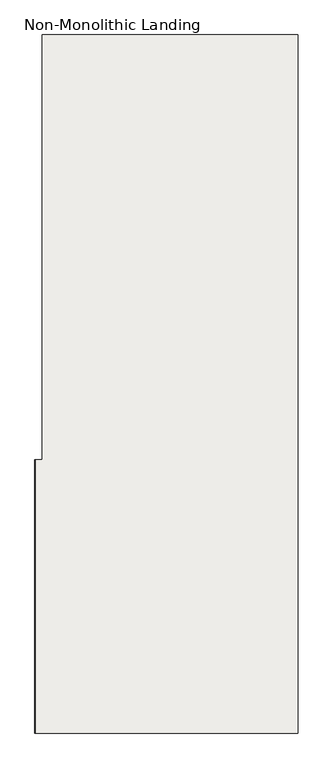
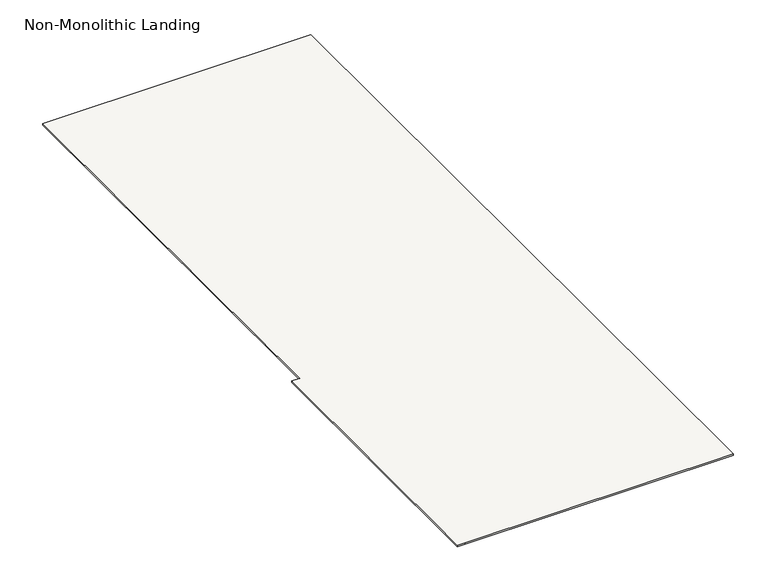
"""IFC4 building model written with IfcOpenShell, lengths in millimetres: slab geometry, Non-Monolithic Landing."""

from ifc_helpers import new_model, si_unit, origin, place, context, project, spatial, faceted_brep, source, transform, mapped, element, save


def non_monolithic_landing_37a11202(model_context):
    return source(origin(), model_context, "Body", "Brep", [
        faceted_brep([(-13356.0599092, 11395.4345331, 28470.5882353), (-13356.9099092, 11395.4345331, 28464.5882353), (-13356.9099092, 10220.4345331, 28464.5882353), (-13356.0599092, 10220.4345331, 28470.5882353), (-13325.0, 12030.4345331, 28470.5882353), (-13325.0, 11395.4345331, 28470.5882353), (-13325.0, 10220.4345331, 28470.5882353), (-12225.0, 10220.4345331, 28470.5882353), (-12225.0, 13220.4345331, 28470.5882353), (-13325.0, 13220.4345331, 28470.5882353), (-13325.0, 11395.4345331, 28464.5882353), (-13325.0, 12030.4345331, 28464.5882353), (-13324.15, 12030.4345331, 28464.5882353), (-13324.15, 13220.4345331, 28464.5882353), (-12225.0, 13220.4345331, 28464.5882353), (-12225.0, 10220.4345331, 28464.5882353), (-13325.0, 10220.4345331, 28464.5882353)], [[[0, 1, 2, 3]], [[4, 5, 0, 3, 6, 7, 8, 9]], [[10, 11, 12, 13, 14, 15, 16, 2, 1]], [[5, 4, 11, 10]], [[0, 5, 10, 1]], [[6, 3, 2, 16]], [[7, 6, 16, 15]], [[8, 7, 15, 14]], [[9, 8, 14, 13]], [[4, 12, 11]], [[12, 4, 9, 13]]]),
    ])


if __name__ == "__main__":
    model = new_model("IFC4")
    model_context = context("Model", 3, world=origin())
    ifc_project = project(units=[si_unit("LENGTHUNIT", "METRE", prefix="MILLI")], contexts=[model_context])
    site = spatial("IfcSite", under=ifc_project)
    building = spatial("IfcBuilding", under=site)
    placement = place(None, origin())
    non_monolithic_landing_shape = non_monolithic_landing_37a11202(model_context)
    element("IfcSlab", 1, ObjectType="Non-Monolithic Landing", at=placement, inside=building, context=model_context, shape_type="MappedRepresentation", body=[
        mapped(non_monolithic_landing_shape, transform((0.0, 0.0, 0.0), x_axis=(1.0, 0.0, 0.0), y_axis=(0.0, 1.0, 0.0), z_axis=(0.0, 0.0, 1.0))),
    ])
    save(model, "model.ifc")

# Revit data of these elements
# Element 1 (IfcSlab, "Non-Monolithic Landing")
#   Materials on its faces: "Steel, Paint Finish, Dark Gray"
# Materials
#   "Steel, Paint Finish, Dark Gray": class "Metal", colour RGB 89 89 89, transparency 0, Description = "Steel, paint finish, dark gray, glossy", Cost = 0
